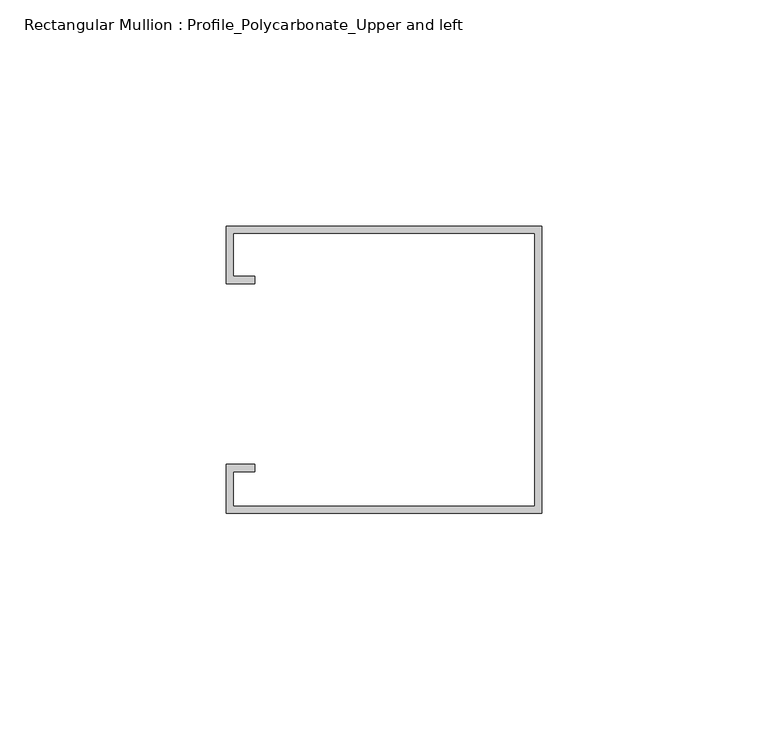
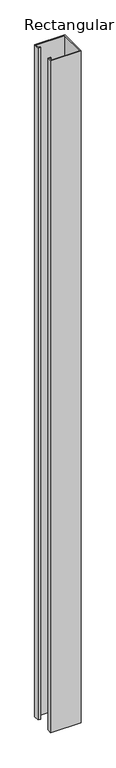
"""IFC4 building model written with IfcOpenShell, lengths in millimetres: member geometry, Rectangular Mullion : Profile_Polycarbonate_Upper and left."""

from ifc_helpers import new_model, si_unit, frame, origin, place, context, project, spatial, polyline, outline, extrude, source, transform, mapped, element, save


def rectangular_mullion_profile_polycarbonate_upper_and_left_b4e19c76(model_context):
    return source(origin(), model_context, "Body", "SweptSolid", [
        extrude(outline(polyline([(0.0, 32.7), (0.0, -30.8), (-69.85, -30.8), (-69.85, -20.0), (-63.5, -20.0), (-63.5, -21.5875), (-68.2625, -21.5875), (-68.2625, -29.2125), (-1.5875, -29.2125), (-1.5875, 31.1125), (-68.2625, 31.1125), (-68.2625, 21.5875), (-63.5, 21.5875), (-63.5, 20.0), (-69.85, 20.0), (-69.85, 32.7), (0.0, 32.7)])), frame((0.0, 0.0, -1638.3), z_axis=(0.0, 0.0, 1.0), x_axis=(1.0, 0.0, 0.0)), (0.0, 0.0, 1.0), 1638.3),
    ])


if __name__ == "__main__":
    model = new_model("IFC4")
    model_context = context("Model", 3, world=origin())
    ifc_project = project(units=[si_unit("LENGTHUNIT", "METRE", prefix="MILLI")], contexts=[model_context])
    site = spatial("IfcSite", under=ifc_project)
    building = spatial("IfcBuilding", under=site)
    placement = place(None, origin())
    rectangular_mullion_profile_polycarbonate_upper_and_left_shape = rectangular_mullion_profile_polycarbonate_upper_and_left_b4e19c76(model_context)
    element("IfcMember", 1, ObjectType="Rectangular Mullion : Profile_Polycarbonate_Upper and left", at=placement, inside=building, context=model_context, shape_type="MappedRepresentation", body=[
        mapped(rectangular_mullion_profile_polycarbonate_upper_and_left_shape, transform((0.0, 0.0, 0.0), x_axis=(1.0, 0.0, 0.0), y_axis=(0.0, 1.0, 0.0), z_axis=(0.0, 0.0, 1.0))),
    ])
    save(model, "model.ifc")

# Revit data of these elements
# Type "Rectangular Mullion : Profile_Polycarbonate_Upper and left"
#   built-in parameter 1007322 = 0.208333 (stored number, unit not read)
#   built-in parameter 1007321 = 0.00520833 (stored number, unit not read)
#   built-in parameter 1007320 = 0 (stored number, unit not read)
# Element 1 (IfcMember, "Rectangular Mullion : Profile_Polycarbonate_Upper and left")
#   Materials on its faces: "GALVANIZED UNISTRUT P5500, 1 5/8\" X 2 7/16\" OR ALUM. CHANNEL"
# Materials
#   "GALVANIZED UNISTRUT P5500, 1 5/8\" X 2 7/16\" OR ALUM. CHANNEL": class "Metal", colour RGB 244 244 244, transparency 0, Description = "Aluminum 6061", Cost = 0
